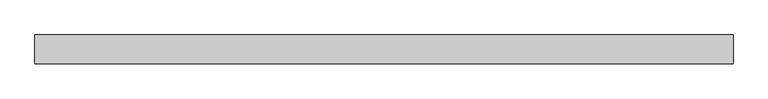
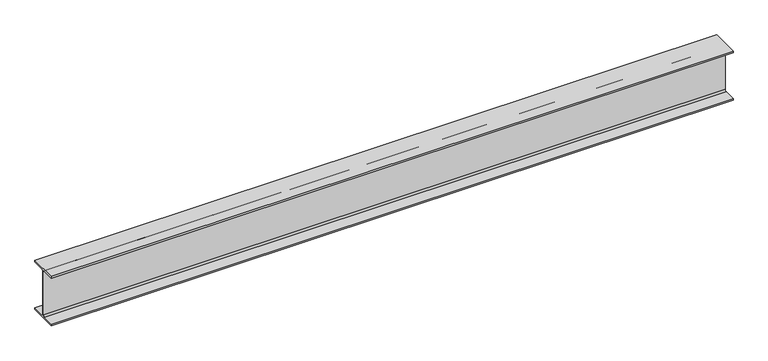
"""IFC4 building model written with IfcOpenShell, lengths in millimetres: beam geometry, Old_Steel Beam_H-KSD3502 : H_SB_ASB_H-390×300x10x16."""

from ifc_helpers import new_model, si_unit, point, frame, frame_2d, origin, place, context, project, spatial, polyline, circle_curve, trimmed, segment, composite_curve, outline, extrude, source, transform, mapped, element, save


def beam_af2d9473(model_context):
    return source(origin(), model_context, "Body", "SweptSolid", [
        extrude(outline(composite_curve([segment(polyline([(82.5, -141.5), (82.5, -151.7), (-82.5, -151.7), (-82.5, -141.5), (-11.9, -141.5)]), True, "CONTINUOUS"), segment(trimmed(circle_curve(frame_2d((-11.9, -132.6)), 8.9), [point((-11.9, -141.5))], [point((-3.0, -132.6))], True, "CARTESIAN"), True, "CONTINUOUS"), segment(polyline([(-3.0, -132.6), (-3.0, 132.6)]), True, "CONTINUOUS"), segment(trimmed(circle_curve(frame_2d((-11.9, 132.6)), 8.9), [point((-3.0, 132.6))], [point((-11.9, 141.5))], True, "CARTESIAN"), True, "CONTINUOUS"), segment(polyline([(-11.9, 141.5), (-82.5, 141.5), (-82.5, 151.7), (82.5, 151.7), (82.5, 141.5), (11.9, 141.5)]), True, "CONTINUOUS"), segment(trimmed(circle_curve(frame_2d((11.9, 132.6)), 8.9), [point((11.9, 141.5))], [point((3.0, 132.6))], True, "CARTESIAN"), True, "CONTINUOUS"), segment(polyline([(3.0, 132.6), (3.0, -132.6)]), True, "CONTINUOUS"), segment(trimmed(circle_curve(frame_2d((11.9, -132.6)), 8.9), [point((3.0, -132.6))], [point((11.9, -141.5))], True, "CARTESIAN"), True, "CONTINUOUS"), segment(polyline([(11.9, -141.5), (82.5, -141.5)]), True, "CONTINUOUS")], self_intersect=False)), frame((-1987.2999994, 0.0, 0.0), z_axis=(1.0, 0.0, 0.0), x_axis=(0.0, 1.0, 0.0)), (0.0, 0.0, 1.0), 3974.5999988),
    ])


if __name__ == "__main__":
    model = new_model("IFC4")
    model_context = context("Model", 3, world=origin())
    ifc_project = project(units=[si_unit("LENGTHUNIT", "METRE", prefix="MILLI")], contexts=[model_context])
    site = spatial("IfcSite", under=ifc_project)
    building = spatial("IfcBuilding", under=site)
    placement = place(None, origin())
    beam_shape = beam_af2d9473(model_context)
    element("IfcBeam", 1, ObjectType="Old_Steel Beam_H-KSD3502 : H_SB_ASB_H-390×300x10x16", at=placement, inside=building, context=model_context, shape_type="MappedRepresentation", body=[
        mapped(beam_shape, transform((0.0, 0.0, 0.0), x_axis=(1.0, 0.0, 0.0), y_axis=(0.0, 1.0, 0.0), z_axis=(0.0, 0.0, 1.0))),
    ])
    save(model, "model.ifc")

# Revit data of these elements
# Type "Old_Steel Beam_H-KSD3502 : H_SB_ASB_H-390×300x10x16"
#   Width = 30.0 cm
#   Web Thickness = 1.0 cm
#   Web Fillet = 2.2 cm
#   Warping Constant = 2517770.0 cm⁶
#   Torsional Moment of Inertia = 94.3867 cm⁴
#   Torsional Modulus = 1.0 cm³
#   Section Area = 136.0 cm²
#   Plastic Modulus weak axis = 733.0 cm³
#   Plastic Modulus strong axis = 2190.0 cm³
#   Perimeter = 1.92 m²/m
#   Nominal Weight = 107.00 kgf/m
#   Moment of Inertia weak axis = 7210.00 cm⁴
#   Moment of Inertia strong axis = 38700.00 cm⁴
#   Height = 39.0 cm
#   Flange Thickness = 1.6 cm
#   Elastic Modulus weak axis = 481.0 cm³
#   Elastic Modulus strong axis = 1980.0 cm³
#   Centroid Vertical = 19.5 cm
#   Centroid Horizontal = 15.0 cm
#   Length [instance default] = 1.5240 m
#   Structural Material [instance default] = Steel, 45-345
#   Assembly Code = ""
# Element 1 (IfcBeam, "Old_Steel Beam_H-KSD3502 : H_SB_ASB_H-390×300x10x16")
#   Structural Material = none
# Materials
#   "Steel, 45-345": class "Metal", colour RGB 189 187 185, transparency 0, Description = "Steel 345 MPa", Cost = 0
